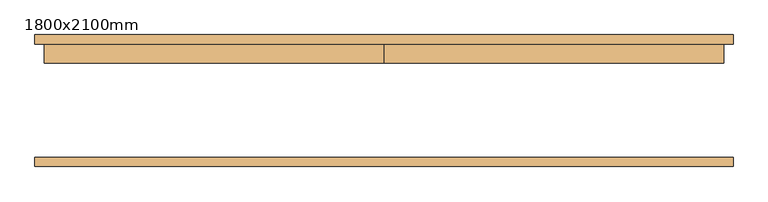
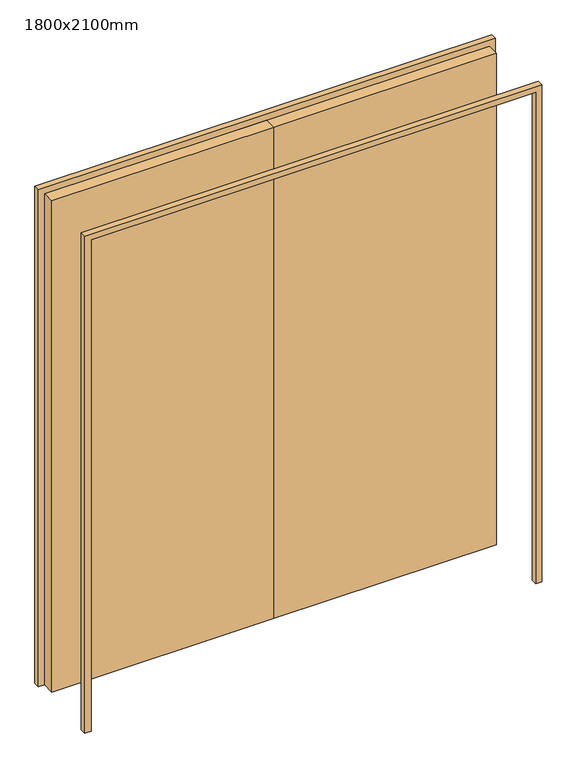
"""IFC4 building model written with IfcOpenShell, lengths in millimetres: door geometry, WWm-DoubleSolid-Flush : 1800x2100mm."""

import ifcopenshell
import ifcopenshell.guid

model = None  # the IFC model being written
_history = None  # IfcOwnerHistory: only IFC2X3 demands one
_inside = {}  # id of a spatial element -> (the spatial element, [elements in it])
_under = {}  # id of a project, library or spatial element -> (it, [spatial elements below it])
_declared = {}  # id of a project -> (the project, [libraries it declares])
_typed = {}  # id of a type object -> (the type object, [elements of that type])
_made_of = {}  # id of a material, layer set ... -> (it, [elements and type objects made of it])


def new_model(schema):
    """Start an empty IFC model of exactly this schema.

    Asked for "IFC4X3", IfcOpenShell would pick the latest addendum, in which some entities
    have other attributes; the version numbers below select the first issue.
    IFC2X3 requires an IfcOwnerHistory on every rooted entity: one is made here for all.
    """
    global model, _history
    if schema == "IFC4X3":
        model = ifcopenshell.file(schema_version=(4, 3, 0, 0))
    else:
        model = ifcopenshell.file(schema=schema)
    _inside.clear()
    _under.clear()
    _declared.clear()
    _typed.clear()
    _made_of.clear()
    _history = None
    if model.schema == "IFC2X3":
        org = make("IfcOrganization", Name="unknown")
        user = make(
            "IfcPersonAndOrganization",
            ThePerson=make("IfcPerson", FamilyName="unknown"),
            TheOrganization=org,
        )
        app = make(
            "IfcApplication",
            ApplicationDeveloper=org,
            Version="unknown",
            ApplicationFullName="unknown",
            ApplicationIdentifier="unknown",
        )
        _history = make(
            "IfcOwnerHistory",
            OwningUser=user,
            OwningApplication=app,
            ChangeAction="ADDED",
            CreationDate=0,
        )
    return model


def make(cls, **values):
    """One entity of the class cls with the attributes given. An attribute that is None is left unset."""
    return model.create_entity(
        cls, **{name: value for name, value in values.items() if value is not None}
    )


def rooted(cls, **values):
    """An entity with a GlobalId (a new one), such as an element, a storey or a relation."""
    return make(cls, GlobalId=ifcopenshell.guid.new(), OwnerHistory=_history, **values)


def si_unit(unit_type, name, prefix=None):
    """IfcSIUnit, for example si_unit("LENGTHUNIT", "METRE", prefix="MILLI")."""
    return make("IfcSIUnit", UnitType=unit_type, Prefix=prefix, Name=name)


def assignment(units):
    """IfcUnitAssignment: the units of a project."""
    return None if units is None else make("IfcUnitAssignment", Units=units)


def point(xyz):
    """IfcCartesianPoint."""
    return None if xyz is None else make("IfcCartesianPoint", Coordinates=xyz)


def direction(xyz):
    """IfcDirection."""
    return None if xyz is None else make("IfcDirection", DirectionRatios=xyz)


def frame(location, z_axis=None, x_axis=None):
    """IfcAxis2Placement3D, a coordinate frame: its origin and axes. An axis left out is left unset."""
    return make(
        "IfcAxis2Placement3D",
        Location=point(location),
        Axis=direction(z_axis),
        RefDirection=direction(x_axis),
    )


def origin():
    """The frame at (0, 0, 0) with its axes left unset."""
    return frame((0.0, 0.0, 0.0))


def origin_with_axes():
    """The frame at (0, 0, 0) with the z axis (0, 0, 1) and the x axis (1, 0, 0) written out."""
    return frame((0.0, 0.0, 0.0), z_axis=(0.0, 0.0, 1.0), x_axis=(1.0, 0.0, 0.0))


def place(relative_to, where):
    """IfcLocalPlacement: puts the frame where relative to a parent placement (None: the world)."""
    return make(
        "IfcLocalPlacement", PlacementRelTo=relative_to, RelativePlacement=where
    )


def context(
    kind, dimensions, precision=None, world=None, true_north=None, identifier=None
):
    """IfcGeometricRepresentationContext, for example the 3D "Model" context."""
    return make(
        "IfcGeometricRepresentationContext",
        ContextIdentifier=identifier,
        ContextType=kind,
        CoordinateSpaceDimension=dimensions,
        Precision=precision,
        WorldCoordinateSystem=world,
        TrueNorth=true_north,
    )


def project(units=None, contexts=None):
    """IfcProject with its units and contexts."""
    return rooted(
        "IfcProject",
        Name="project",
        RepresentationContexts=contexts,
        UnitsInContext=assignment(units),
    )


def spatial(cls, under=None, at=None, **own):
    """A site, building, storey or space (cls), placed at a placement, below another one or the project."""
    s = rooted(cls, ObjectPlacement=at, **own)
    if under is not None:
        _under.setdefault(under.id(), (under, []))[1].append(s)
    return s


def polyline(points):
    """IfcPolyline through the points."""
    return make("IfcPolyline", Points=[point(p) for p in points])


def outline(outer, holes=None, kind="AREA"):
    """IfcArbitraryClosedProfileDef: a profile drawn as a closed curve; with holes, ...WithVoids."""
    if holes is None:
        return make("IfcArbitraryClosedProfileDef", ProfileType=kind, OuterCurve=outer)
    return make(
        "IfcArbitraryProfileDefWithVoids",
        ProfileType=kind,
        OuterCurve=outer,
        InnerCurves=holes,
    )


def extrude(swept, where, along, depth):
    """IfcExtrudedAreaSolid: the profile swept, set in the frame where, extruded along a direction by depth."""
    return make(
        "IfcExtrudedAreaSolid",
        SweptArea=swept,
        Position=where,
        ExtrudedDirection=direction(along),
        Depth=depth,
    )


def shape(context_of_items, identifier, shape_type, items):
    """IfcShapeRepresentation: the items that make up one representation, for example the "Body"."""
    return make(
        "IfcShapeRepresentation",
        ContextOfItems=context_of_items,
        RepresentationIdentifier=identifier,
        RepresentationType=shape_type,
        Items=items,
    )


def source(mapping_origin, context_of_items, identifier, shape_type, items):
    """IfcRepresentationMap: a shape defined once, which mapped items show again and again."""
    return make(
        "IfcRepresentationMap",
        MappingOrigin=mapping_origin,
        MappedRepresentation=shape(context_of_items, identifier, shape_type, items),
    )


def transform(
    local_origin,
    x_axis=None,
    y_axis=None,
    z_axis=None,
    scale=None,
    scale2=None,
    scale3=None,
    uniform=True,
):
    """IfcCartesianTransformationOperator3D, or its non-uniform kind. x_axis, y_axis, z_axis: its Axis1, 2, 3."""
    if uniform:
        return make(
            "IfcCartesianTransformationOperator3D",
            Axis1=direction(x_axis),
            Axis2=direction(y_axis),
            LocalOrigin=point(local_origin),
            Scale=scale,
            Axis3=direction(z_axis),
        )
    return make(
        "IfcCartesianTransformationOperator3DnonUniform",
        Axis1=direction(x_axis),
        Axis2=direction(y_axis),
        LocalOrigin=point(local_origin),
        Scale=scale,
        Axis3=direction(z_axis),
        Scale2=scale2,
        Scale3=scale3,
    )


def mapped(mapping_source, mapping_target):
    """IfcMappedItem: shows the shape of a source again, moved by a transform."""
    return make(
        "IfcMappedItem", MappingSource=mapping_source, MappingTarget=mapping_target
    )


def made_of(thing, what):
    """Note that an element or type object is made of a material, layer set ...; save() writes the relation."""
    if what is not None:
        _made_of.setdefault(what.id(), (what, []))[1].append(thing)
    return thing


def element(
    cls,
    number,
    at=None,
    inside=None,
    cuts=None,
    type_object=None,
    material=None,
    context=None,
    identifier="Body",
    shape_type=None,
    held_by="IfcProductDefinitionShape",
    body=None,
    shapes=None,
    **own,
):
    """One element of the class cls, such as IfcWall. Its Tag is "e" and its number.

    at: its placement. inside: the storey or other place that contains it. cuts: it is an
    opening in that element (IfcRelVoidsElement). A single representation is given by context,
    identifier, shape_type and body (its items); several are given by shapes. held_by: the class
    of the entity that holds the representations. save() writes the other relations.
    """
    e = rooted(cls, Tag="e%d" % number, ObjectPlacement=at, **own)
    if body is not None:
        shapes = [shape(context, identifier, shape_type, body)]
    if shapes is not None:
        e.Representation = make(held_by, Representations=shapes)
    if inside is not None:
        _inside.setdefault(inside.id(), (inside, []))[1].append(e)
    if cuts is not None:
        rooted(
            "IfcRelVoidsElement", RelatingBuildingElement=cuts, RelatedOpeningElement=e
        )
    if type_object is not None:
        _typed.setdefault(type_object.id(), (type_object, []))[1].append(e)
    return made_of(e, material)


def aggregate(whole, parts):
    """IfcRelAggregates: a whole, such as a stair, and the parts it consists of."""
    return rooted("IfcRelAggregates", RelatingObject=whole, RelatedObjects=parts)


def save(model, path):
    """Write the relations noted so far, then the file.

    IfcRelAggregates (storeys below a building ...), IfcRelContainedInSpatialStructure (elements
    in a storey), IfcRelDefinesByType, IfcRelAssociatesMaterial and IfcRelDeclares: one each for
    every whole, place, type object, material and project.
    """
    for whole, parts in _under.values():
        aggregate(whole, parts)
    for where, things in _inside.values():
        rooted(
            "IfcRelContainedInSpatialStructure",
            RelatedElements=things,
            RelatingStructure=where,
        )
    for kind, things in _typed.values():
        rooted("IfcRelDefinesByType", RelatedObjects=things, RelatingType=kind)
    for what, things in _made_of.values():
        rooted("IfcRelAssociatesMaterial", RelatedObjects=things, RelatingMaterial=what)
    for by, libraries in _declared.values():
        rooted("IfcRelDeclares", RelatingContext=by, RelatedDefinitions=libraries)
    model.write(path)


def door_1800x2100mm_2545e203(model_context):
    return source(origin(), model_context, "Body", "SweptSolid", [
        extrude(outline(polyline([(0.0, 150.0), (900.0, 150.0), (900.0, 100.0), (0.0, 100.0), (0.0, 150.0)])), origin_with_axes(), (0.0, 0.0, 1.0), 2100.0),
        extrude(outline(polyline([(-900.0, 150.0), (0.0, 150.0), (0.0, 100.0), (-900.0, 100.0), (-900.0, 150.0)])), origin_with_axes(), (0.0, 0.0, 1.0), 2100.0),
        extrude(outline(polyline([(2100.0, -900.0), (2100.0, 900.0), (0.0, 900.0), (0.0, 925.0), (2125.0, 925.0), (2125.0, -925.0), (0.0, -925.0), (0.0, -900.0), (2100.0, -900.0)])), frame((0.0, -175.0, 0.0), z_axis=(0.0, 1.0, 0.0), x_axis=(0.0, 0.0, 1.0)), (0.0, 0.0, 1.0), 25.0),
        extrude(outline(polyline([(2100.0, -900.0), (2100.0, 900.0), (0.0, 900.0), (0.0, 925.0), (2125.0, 925.0), (2125.0, -925.0), (0.0, -925.0), (0.0, -900.0), (2100.0, -900.0)])), frame((0.0, 150.0, 0.0), z_axis=(0.0, 1.0, 0.0), x_axis=(0.0, 0.0, 1.0)), (0.0, 0.0, 1.0), 25.0),
    ])


if __name__ == "__main__":
    model = new_model("IFC4")
    model_context = context("Model", 3, world=origin())
    ifc_project = project(units=[si_unit("LENGTHUNIT", "METRE", prefix="MILLI")], contexts=[model_context])
    site = spatial("IfcSite", under=ifc_project)
    building = spatial("IfcBuilding", under=site)
    placement = place(None, origin())
    door_1800x2100mm_shape = door_1800x2100mm_2545e203(model_context)
    element("IfcDoor", 1, ObjectType="WWm-DoubleSolid-Flush : 1800x2100mm", at=placement, inside=building, context=model_context, shape_type="MappedRepresentation", body=[
        mapped(door_1800x2100mm_shape, transform((0.0, 0.0, 0.0), x_axis=(1.0, 0.0, 0.0), y_axis=(0.0, 1.0, 0.0), z_axis=(0.0, 0.0, 1.0))),
    ])
    save(model, "model.ifc")

# Revit data of these elements
# Type "WWm-DoubleSolid-Flush : 1800x2100mm"
#   Type Mark = "EX1-44"
#   Construction Type Id = "MDOOR"
#   Assembly Code = "C1020"
#   Analytic Construction = "Metal"
#   Thickness = 50 mm
#   Thermal Resistance (R) = 0.270117 (m²·K)/W
#   Heat Transfer Coefficient (U) = 3.7021 W/(m²·K)
#   Height = 2100 mm
#   Trim Projection Ext = 25 mm
#   Trim Projection Int = 25 mm
#   Trim Width = 25 mm
#   Width = 1800 mm
#   Not 90 Degree [instance default] = no
#   90 Degree [instance default] = yes
#   Door Material = WW-EC-RGB-White
#   Frame Material = WW-EC-RGB-White
#   Visual Light Transmittance = 0
#   Solar Heat Gain Coefficient = 0
#   Function = (empty or 0)
#   Wall Closure = (empty or 0)
# Element 1 (IfcDoor, "WWm-DoubleSolid-Flush : 1800x2100mm")
#   Materials on its faces: "WW-EC-RGB-White"
# Materials
#   "WW-EC-RGB-White": class "Generic", colour RGB 255 255 255, transparency 0, Comments = "If region requests off-white, swith asset color to RGB 231-228-220", Description = "Generic Color", Cost = 0
